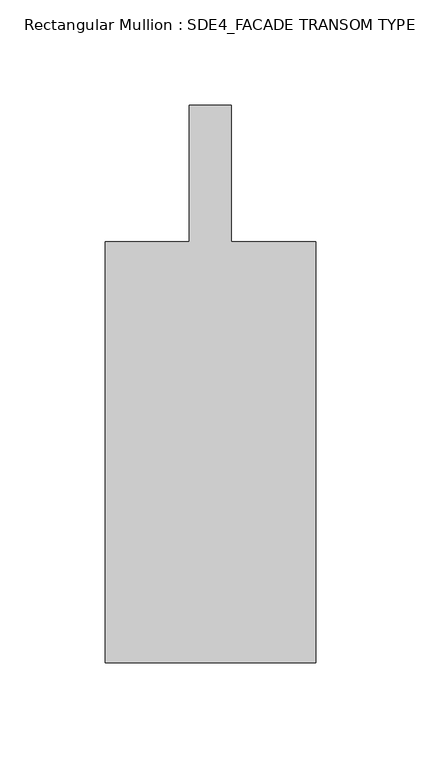
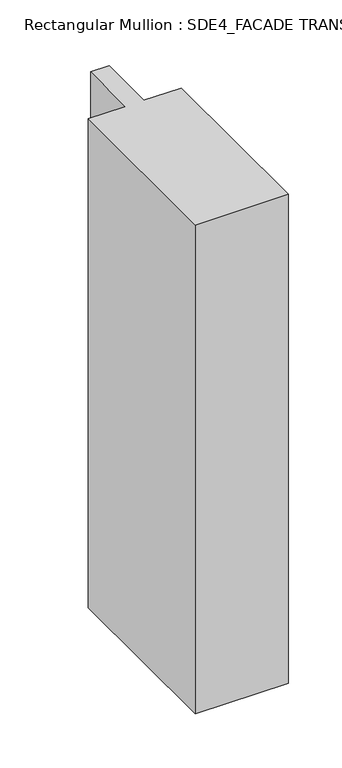
"""IFC4 building model written with IfcOpenShell, lengths in millimetres: member geometry, Rectangular Mullion : SDE4_FACADE TRANSOM TYPE 2."""

import ifcopenshell
import ifcopenshell.guid

model = None  # the IFC model being written
_history = None  # IfcOwnerHistory: only IFC2X3 demands one
_inside = {}  # id of a spatial element -> (the spatial element, [elements in it])
_under = {}  # id of a project, library or spatial element -> (it, [spatial elements below it])
_declared = {}  # id of a project -> (the project, [libraries it declares])
_typed = {}  # id of a type object -> (the type object, [elements of that type])
_made_of = {}  # id of a material, layer set ... -> (it, [elements and type objects made of it])


def new_model(schema):
    """Start an empty IFC model of exactly this schema.

    Asked for "IFC4X3", IfcOpenShell would pick the latest addendum, in which some entities
    have other attributes; the version numbers below select the first issue.
    IFC2X3 requires an IfcOwnerHistory on every rooted entity: one is made here for all.
    """
    global model, _history
    if schema == "IFC4X3":
        model = ifcopenshell.file(schema_version=(4, 3, 0, 0))
    else:
        model = ifcopenshell.file(schema=schema)
    _inside.clear()
    _under.clear()
    _declared.clear()
    _typed.clear()
    _made_of.clear()
    _history = None
    if model.schema == "IFC2X3":
        org = make("IfcOrganization", Name="unknown")
        user = make(
            "IfcPersonAndOrganization",
            ThePerson=make("IfcPerson", FamilyName="unknown"),
            TheOrganization=org,
        )
        app = make(
            "IfcApplication",
            ApplicationDeveloper=org,
            Version="unknown",
            ApplicationFullName="unknown",
            ApplicationIdentifier="unknown",
        )
        _history = make(
            "IfcOwnerHistory",
            OwningUser=user,
            OwningApplication=app,
            ChangeAction="ADDED",
            CreationDate=0,
        )
    return model


def make(cls, **values):
    """One entity of the class cls with the attributes given. An attribute that is None is left unset."""
    return model.create_entity(
        cls, **{name: value for name, value in values.items() if value is not None}
    )


def rooted(cls, **values):
    """An entity with a GlobalId (a new one), such as an element, a storey or a relation."""
    return make(cls, GlobalId=ifcopenshell.guid.new(), OwnerHistory=_history, **values)


def si_unit(unit_type, name, prefix=None):
    """IfcSIUnit, for example si_unit("LENGTHUNIT", "METRE", prefix="MILLI")."""
    return make("IfcSIUnit", UnitType=unit_type, Prefix=prefix, Name=name)


def assignment(units):
    """IfcUnitAssignment: the units of a project."""
    return None if units is None else make("IfcUnitAssignment", Units=units)


def point(xyz):
    """IfcCartesianPoint."""
    return None if xyz is None else make("IfcCartesianPoint", Coordinates=xyz)


def direction(xyz):
    """IfcDirection."""
    return None if xyz is None else make("IfcDirection", DirectionRatios=xyz)


def frame(location, z_axis=None, x_axis=None):
    """IfcAxis2Placement3D, a coordinate frame: its origin and axes. An axis left out is left unset."""
    return make(
        "IfcAxis2Placement3D",
        Location=point(location),
        Axis=direction(z_axis),
        RefDirection=direction(x_axis),
    )


def origin():
    """The frame at (0, 0, 0) with its axes left unset."""
    return frame((0.0, 0.0, 0.0))


def place(relative_to, where):
    """IfcLocalPlacement: puts the frame where relative to a parent placement (None: the world)."""
    return make(
        "IfcLocalPlacement", PlacementRelTo=relative_to, RelativePlacement=where
    )


def context(
    kind, dimensions, precision=None, world=None, true_north=None, identifier=None
):
    """IfcGeometricRepresentationContext, for example the 3D "Model" context."""
    return make(
        "IfcGeometricRepresentationContext",
        ContextIdentifier=identifier,
        ContextType=kind,
        CoordinateSpaceDimension=dimensions,
        Precision=precision,
        WorldCoordinateSystem=world,
        TrueNorth=true_north,
    )


def project(units=None, contexts=None):
    """IfcProject with its units and contexts."""
    return rooted(
        "IfcProject",
        Name="project",
        RepresentationContexts=contexts,
        UnitsInContext=assignment(units),
    )


def spatial(cls, under=None, at=None, **own):
    """A site, building, storey or space (cls), placed at a placement, below another one or the project."""
    s = rooted(cls, ObjectPlacement=at, **own)
    if under is not None:
        _under.setdefault(under.id(), (under, []))[1].append(s)
    return s


def polyline(points):
    """IfcPolyline through the points."""
    return make("IfcPolyline", Points=[point(p) for p in points])


def outline(outer, holes=None, kind="AREA"):
    """IfcArbitraryClosedProfileDef: a profile drawn as a closed curve; with holes, ...WithVoids."""
    if holes is None:
        return make("IfcArbitraryClosedProfileDef", ProfileType=kind, OuterCurve=outer)
    return make(
        "IfcArbitraryProfileDefWithVoids",
        ProfileType=kind,
        OuterCurve=outer,
        InnerCurves=holes,
    )


def extrude(swept, where, along, depth):
    """IfcExtrudedAreaSolid: the profile swept, set in the frame where, extruded along a direction by depth."""
    return make(
        "IfcExtrudedAreaSolid",
        SweptArea=swept,
        Position=where,
        ExtrudedDirection=direction(along),
        Depth=depth,
    )


def shape(context_of_items, identifier, shape_type, items):
    """IfcShapeRepresentation: the items that make up one representation, for example the "Body"."""
    return make(
        "IfcShapeRepresentation",
        ContextOfItems=context_of_items,
        RepresentationIdentifier=identifier,
        RepresentationType=shape_type,
        Items=items,
    )


def source(mapping_origin, context_of_items, identifier, shape_type, items):
    """IfcRepresentationMap: a shape defined once, which mapped items show again and again."""
    return make(
        "IfcRepresentationMap",
        MappingOrigin=mapping_origin,
        MappedRepresentation=shape(context_of_items, identifier, shape_type, items),
    )


def transform(
    local_origin,
    x_axis=None,
    y_axis=None,
    z_axis=None,
    scale=None,
    scale2=None,
    scale3=None,
    uniform=True,
):
    """IfcCartesianTransformationOperator3D, or its non-uniform kind. x_axis, y_axis, z_axis: its Axis1, 2, 3."""
    if uniform:
        return make(
            "IfcCartesianTransformationOperator3D",
            Axis1=direction(x_axis),
            Axis2=direction(y_axis),
            LocalOrigin=point(local_origin),
            Scale=scale,
            Axis3=direction(z_axis),
        )
    return make(
        "IfcCartesianTransformationOperator3DnonUniform",
        Axis1=direction(x_axis),
        Axis2=direction(y_axis),
        LocalOrigin=point(local_origin),
        Scale=scale,
        Axis3=direction(z_axis),
        Scale2=scale2,
        Scale3=scale3,
    )


def mapped(mapping_source, mapping_target):
    """IfcMappedItem: shows the shape of a source again, moved by a transform."""
    return make(
        "IfcMappedItem", MappingSource=mapping_source, MappingTarget=mapping_target
    )


def made_of(thing, what):
    """Note that an element or type object is made of a material, layer set ...; save() writes the relation."""
    if what is not None:
        _made_of.setdefault(what.id(), (what, []))[1].append(thing)
    return thing


def element(
    cls,
    number,
    at=None,
    inside=None,
    cuts=None,
    type_object=None,
    material=None,
    context=None,
    identifier="Body",
    shape_type=None,
    held_by="IfcProductDefinitionShape",
    body=None,
    shapes=None,
    **own,
):
    """One element of the class cls, such as IfcWall. Its Tag is "e" and its number.

    at: its placement. inside: the storey or other place that contains it. cuts: it is an
    opening in that element (IfcRelVoidsElement). A single representation is given by context,
    identifier, shape_type and body (its items); several are given by shapes. held_by: the class
    of the entity that holds the representations. save() writes the other relations.
    """
    e = rooted(cls, Tag="e%d" % number, ObjectPlacement=at, **own)
    if body is not None:
        shapes = [shape(context, identifier, shape_type, body)]
    if shapes is not None:
        e.Representation = make(held_by, Representations=shapes)
    if inside is not None:
        _inside.setdefault(inside.id(), (inside, []))[1].append(e)
    if cuts is not None:
        rooted(
            "IfcRelVoidsElement", RelatingBuildingElement=cuts, RelatedOpeningElement=e
        )
    if type_object is not None:
        _typed.setdefault(type_object.id(), (type_object, []))[1].append(e)
    return made_of(e, material)


def aggregate(whole, parts):
    """IfcRelAggregates: a whole, such as a stair, and the parts it consists of."""
    return rooted("IfcRelAggregates", RelatingObject=whole, RelatedObjects=parts)


def save(model, path):
    """Write the relations noted so far, then the file.

    IfcRelAggregates (storeys below a building ...), IfcRelContainedInSpatialStructure (elements
    in a storey), IfcRelDefinesByType, IfcRelAssociatesMaterial and IfcRelDeclares: one each for
    every whole, place, type object, material and project.
    """
    for whole, parts in _under.values():
        aggregate(whole, parts)
    for where, things in _inside.values():
        rooted(
            "IfcRelContainedInSpatialStructure",
            RelatedElements=things,
            RelatingStructure=where,
        )
    for kind, things in _typed.values():
        rooted("IfcRelDefinesByType", RelatedObjects=things, RelatingType=kind)
    for what, things in _made_of.values():
        rooted("IfcRelAssociatesMaterial", RelatedObjects=things, RelatingMaterial=what)
    for by, libraries in _declared.values():
        rooted("IfcRelDeclares", RelatingContext=by, RelatedDefinitions=libraries)
    model.write(path)


def rectangular_mullion_sde4_facade_transom_type_2_b007ec8b(model_context):
    return source(origin(), model_context, "Body", "SweptSolid", [
        extrude(outline(polyline([(50.0, -132.5), (-50.0, -132.5), (-50.0, 67.5), (-10.0, 67.5), (-10.0, 132.5), (10.0, 132.5), (10.0, 67.5), (50.0, 67.5), (50.0, -132.5)])), frame((0.0, 0.0, -557.9029609), z_axis=(0.0, 0.0, 1.0), x_axis=(1.0, 0.0, 0.0)), (0.0, 0.0, 1.0), 557.9029609),
    ])


if __name__ == "__main__":
    model = new_model("IFC4")
    model_context = context("Model", 3, world=origin())
    ifc_project = project(units=[si_unit("LENGTHUNIT", "METRE", prefix="MILLI")], contexts=[model_context])
    site = spatial("IfcSite", under=ifc_project)
    building = spatial("IfcBuilding", under=site)
    placement = place(None, origin())
    rectangular_mullion_sde4_facade_transom_type_2_shape = rectangular_mullion_sde4_facade_transom_type_2_b007ec8b(model_context)
    element("IfcMember", 1, ObjectType="Rectangular Mullion : SDE4_FACADE TRANSOM TYPE 2", at=placement, inside=building, context=model_context, shape_type="MappedRepresentation", body=[
        mapped(rectangular_mullion_sde4_facade_transom_type_2_shape, transform((0.0, 0.0, 0.0), x_axis=(1.0, 0.0, 0.0), y_axis=(0.0, 1.0, 0.0), z_axis=(0.0, 0.0, 1.0))),
    ])
    save(model, "model.ifc")

# Revit data of these elements
# Type "Rectangular Mullion : SDE4_FACADE TRANSOM TYPE 2"
#   built-in parameter 1007322 = 0.869423 (stored number, unit not read)
#   built-in parameter 1007321 = 0.164042 (stored number, unit not read)
#   built-in parameter 1007320 = 0.164042 (stored number, unit not read)
